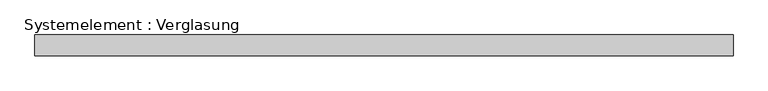
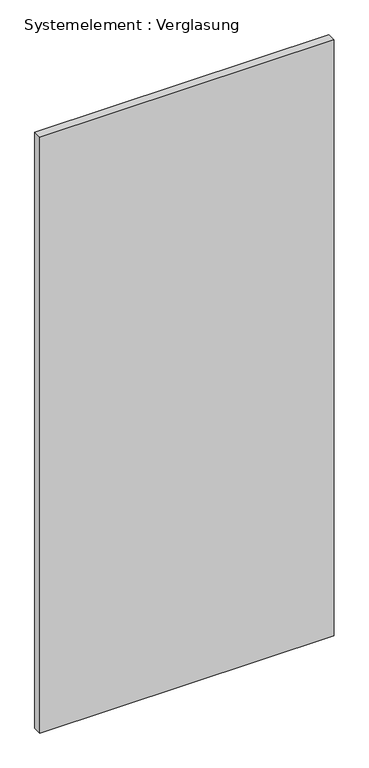
"""IFC4 building model written with IfcOpenShell, lengths in millimetres: plate geometry, Systemelement : Verglasung."""

import ifcopenshell
import ifcopenshell.guid

model = None  # the IFC model being written
_history = None  # IfcOwnerHistory: only IFC2X3 demands one
_inside = {}  # id of a spatial element -> (the spatial element, [elements in it])
_under = {}  # id of a project, library or spatial element -> (it, [spatial elements below it])
_declared = {}  # id of a project -> (the project, [libraries it declares])
_typed = {}  # id of a type object -> (the type object, [elements of that type])
_made_of = {}  # id of a material, layer set ... -> (it, [elements and type objects made of it])


def new_model(schema):
    """Start an empty IFC model of exactly this schema.

    Asked for "IFC4X3", IfcOpenShell would pick the latest addendum, in which some entities
    have other attributes; the version numbers below select the first issue.
    IFC2X3 requires an IfcOwnerHistory on every rooted entity: one is made here for all.
    """
    global model, _history
    if schema == "IFC4X3":
        model = ifcopenshell.file(schema_version=(4, 3, 0, 0))
    else:
        model = ifcopenshell.file(schema=schema)
    _inside.clear()
    _under.clear()
    _declared.clear()
    _typed.clear()
    _made_of.clear()
    _history = None
    if model.schema == "IFC2X3":
        org = make("IfcOrganization", Name="unknown")
        user = make(
            "IfcPersonAndOrganization",
            ThePerson=make("IfcPerson", FamilyName="unknown"),
            TheOrganization=org,
        )
        app = make(
            "IfcApplication",
            ApplicationDeveloper=org,
            Version="unknown",
            ApplicationFullName="unknown",
            ApplicationIdentifier="unknown",
        )
        _history = make(
            "IfcOwnerHistory",
            OwningUser=user,
            OwningApplication=app,
            ChangeAction="ADDED",
            CreationDate=0,
        )
    return model


def make(cls, **values):
    """One entity of the class cls with the attributes given. An attribute that is None is left unset."""
    return model.create_entity(
        cls, **{name: value for name, value in values.items() if value is not None}
    )


def rooted(cls, **values):
    """An entity with a GlobalId (a new one), such as an element, a storey or a relation."""
    return make(cls, GlobalId=ifcopenshell.guid.new(), OwnerHistory=_history, **values)


def si_unit(unit_type, name, prefix=None):
    """IfcSIUnit, for example si_unit("LENGTHUNIT", "METRE", prefix="MILLI")."""
    return make("IfcSIUnit", UnitType=unit_type, Prefix=prefix, Name=name)


def assignment(units):
    """IfcUnitAssignment: the units of a project."""
    return None if units is None else make("IfcUnitAssignment", Units=units)


def point(xyz):
    """IfcCartesianPoint."""
    return None if xyz is None else make("IfcCartesianPoint", Coordinates=xyz)


def direction(xyz):
    """IfcDirection."""
    return None if xyz is None else make("IfcDirection", DirectionRatios=xyz)


def frame(location, z_axis=None, x_axis=None):
    """IfcAxis2Placement3D, a coordinate frame: its origin and axes. An axis left out is left unset."""
    return make(
        "IfcAxis2Placement3D",
        Location=point(location),
        Axis=direction(z_axis),
        RefDirection=direction(x_axis),
    )


def origin():
    """The frame at (0, 0, 0) with its axes left unset."""
    return frame((0.0, 0.0, 0.0))


def origin_with_axes():
    """The frame at (0, 0, 0) with the z axis (0, 0, 1) and the x axis (1, 0, 0) written out."""
    return frame((0.0, 0.0, 0.0), z_axis=(0.0, 0.0, 1.0), x_axis=(1.0, 0.0, 0.0))


def place(relative_to, where):
    """IfcLocalPlacement: puts the frame where relative to a parent placement (None: the world)."""
    return make(
        "IfcLocalPlacement", PlacementRelTo=relative_to, RelativePlacement=where
    )


def context(
    kind, dimensions, precision=None, world=None, true_north=None, identifier=None
):
    """IfcGeometricRepresentationContext, for example the 3D "Model" context."""
    return make(
        "IfcGeometricRepresentationContext",
        ContextIdentifier=identifier,
        ContextType=kind,
        CoordinateSpaceDimension=dimensions,
        Precision=precision,
        WorldCoordinateSystem=world,
        TrueNorth=true_north,
    )


def project(units=None, contexts=None):
    """IfcProject with its units and contexts."""
    return rooted(
        "IfcProject",
        Name="project",
        RepresentationContexts=contexts,
        UnitsInContext=assignment(units),
    )


def spatial(cls, under=None, at=None, **own):
    """A site, building, storey or space (cls), placed at a placement, below another one or the project."""
    s = rooted(cls, ObjectPlacement=at, **own)
    if under is not None:
        _under.setdefault(under.id(), (under, []))[1].append(s)
    return s


def polyline(points):
    """IfcPolyline through the points."""
    return make("IfcPolyline", Points=[point(p) for p in points])


def outline(outer, holes=None, kind="AREA"):
    """IfcArbitraryClosedProfileDef: a profile drawn as a closed curve; with holes, ...WithVoids."""
    if holes is None:
        return make("IfcArbitraryClosedProfileDef", ProfileType=kind, OuterCurve=outer)
    return make(
        "IfcArbitraryProfileDefWithVoids",
        ProfileType=kind,
        OuterCurve=outer,
        InnerCurves=holes,
    )


def extrude(swept, where, along, depth):
    """IfcExtrudedAreaSolid: the profile swept, set in the frame where, extruded along a direction by depth."""
    return make(
        "IfcExtrudedAreaSolid",
        SweptArea=swept,
        Position=where,
        ExtrudedDirection=direction(along),
        Depth=depth,
    )


def shape(context_of_items, identifier, shape_type, items):
    """IfcShapeRepresentation: the items that make up one representation, for example the "Body"."""
    return make(
        "IfcShapeRepresentation",
        ContextOfItems=context_of_items,
        RepresentationIdentifier=identifier,
        RepresentationType=shape_type,
        Items=items,
    )


def source(mapping_origin, context_of_items, identifier, shape_type, items):
    """IfcRepresentationMap: a shape defined once, which mapped items show again and again."""
    return make(
        "IfcRepresentationMap",
        MappingOrigin=mapping_origin,
        MappedRepresentation=shape(context_of_items, identifier, shape_type, items),
    )


def transform(
    local_origin,
    x_axis=None,
    y_axis=None,
    z_axis=None,
    scale=None,
    scale2=None,
    scale3=None,
    uniform=True,
):
    """IfcCartesianTransformationOperator3D, or its non-uniform kind. x_axis, y_axis, z_axis: its Axis1, 2, 3."""
    if uniform:
        return make(
            "IfcCartesianTransformationOperator3D",
            Axis1=direction(x_axis),
            Axis2=direction(y_axis),
            LocalOrigin=point(local_origin),
            Scale=scale,
            Axis3=direction(z_axis),
        )
    return make(
        "IfcCartesianTransformationOperator3DnonUniform",
        Axis1=direction(x_axis),
        Axis2=direction(y_axis),
        LocalOrigin=point(local_origin),
        Scale=scale,
        Axis3=direction(z_axis),
        Scale2=scale2,
        Scale3=scale3,
    )


def mapped(mapping_source, mapping_target):
    """IfcMappedItem: shows the shape of a source again, moved by a transform."""
    return make(
        "IfcMappedItem", MappingSource=mapping_source, MappingTarget=mapping_target
    )


def made_of(thing, what):
    """Note that an element or type object is made of a material, layer set ...; save() writes the relation."""
    if what is not None:
        _made_of.setdefault(what.id(), (what, []))[1].append(thing)
    return thing


def element(
    cls,
    number,
    at=None,
    inside=None,
    cuts=None,
    type_object=None,
    material=None,
    context=None,
    identifier="Body",
    shape_type=None,
    held_by="IfcProductDefinitionShape",
    body=None,
    shapes=None,
    **own,
):
    """One element of the class cls, such as IfcWall. Its Tag is "e" and its number.

    at: its placement. inside: the storey or other place that contains it. cuts: it is an
    opening in that element (IfcRelVoidsElement). A single representation is given by context,
    identifier, shape_type and body (its items); several are given by shapes. held_by: the class
    of the entity that holds the representations. save() writes the other relations.
    """
    e = rooted(cls, Tag="e%d" % number, ObjectPlacement=at, **own)
    if body is not None:
        shapes = [shape(context, identifier, shape_type, body)]
    if shapes is not None:
        e.Representation = make(held_by, Representations=shapes)
    if inside is not None:
        _inside.setdefault(inside.id(), (inside, []))[1].append(e)
    if cuts is not None:
        rooted(
            "IfcRelVoidsElement", RelatingBuildingElement=cuts, RelatedOpeningElement=e
        )
    if type_object is not None:
        _typed.setdefault(type_object.id(), (type_object, []))[1].append(e)
    return made_of(e, material)


def aggregate(whole, parts):
    """IfcRelAggregates: a whole, such as a stair, and the parts it consists of."""
    return rooted("IfcRelAggregates", RelatingObject=whole, RelatedObjects=parts)


def save(model, path):
    """Write the relations noted so far, then the file.

    IfcRelAggregates (storeys below a building ...), IfcRelContainedInSpatialStructure (elements
    in a storey), IfcRelDefinesByType, IfcRelAssociatesMaterial and IfcRelDeclares: one each for
    every whole, place, type object, material and project.
    """
    for whole, parts in _under.values():
        aggregate(whole, parts)
    for where, things in _inside.values():
        rooted(
            "IfcRelContainedInSpatialStructure",
            RelatedElements=things,
            RelatingStructure=where,
        )
    for kind, things in _typed.values():
        rooted("IfcRelDefinesByType", RelatedObjects=things, RelatingType=kind)
    for what, things in _made_of.values():
        rooted("IfcRelAssociatesMaterial", RelatedObjects=things, RelatingMaterial=what)
    for by, libraries in _declared.values():
        rooted("IfcRelDeclares", RelatingContext=by, RelatedDefinitions=libraries)
    model.write(path)


def systemelement_verglasung_598f1f79(model_context):
    return source(origin(), model_context, "Body", "SweptSolid", [
        extrude(outline(polyline([(504.9886524, -15.0), (-504.9886524, -15.0), (-504.9886524, 15.0), (504.9886524, 15.0), (504.9886524, -15.0)])), origin_with_axes(), (0.0, 0.0, 1.0), 2160.0),
    ])


if __name__ == "__main__":
    model = new_model("IFC4")
    model_context = context("Model", 3, world=origin())
    ifc_project = project(units=[si_unit("LENGTHUNIT", "METRE", prefix="MILLI")], contexts=[model_context])
    site = spatial("IfcSite", under=ifc_project)
    building = spatial("IfcBuilding", under=site)
    placement = place(None, origin())
    systemelement_verglasung_shape = systemelement_verglasung_598f1f79(model_context)
    element("IfcPlate", 1, ObjectType="Systemelement : Verglasung", at=placement, inside=building, context=model_context, shape_type="MappedRepresentation", body=[
        mapped(systemelement_verglasung_shape, transform((0.0, 0.0, 0.0), x_axis=(1.0, 0.0, 0.0), y_axis=(0.0, 1.0, 0.0), z_axis=(0.0, 0.0, 1.0))),
    ])
    save(model, "model.ifc")

# Revit data of these elements
# Type "Systemelement : Verglasung"
#   Construction Type Id = "GSP4R"
#   Analytic Construction = "1/8 Zoll Pilkington-Verglasung einfach"
#   Visual Light Transmittance = 0.9
#   Solar Heat Gain Coefficient = 0.86
#   Heat Transfer Coefficient (U) = 6.7069 W/(m²·K)
# Element 1 (IfcPlate, "Systemelement : Verglasung")
#   Materials on its faces: "Glas"
# Materials
#   "Glas": class "Glas", colour RGB 0 0 255, transparency 0.75, Comments = "Render-Darstellung nicht aktualisiert ", Cost = 0
